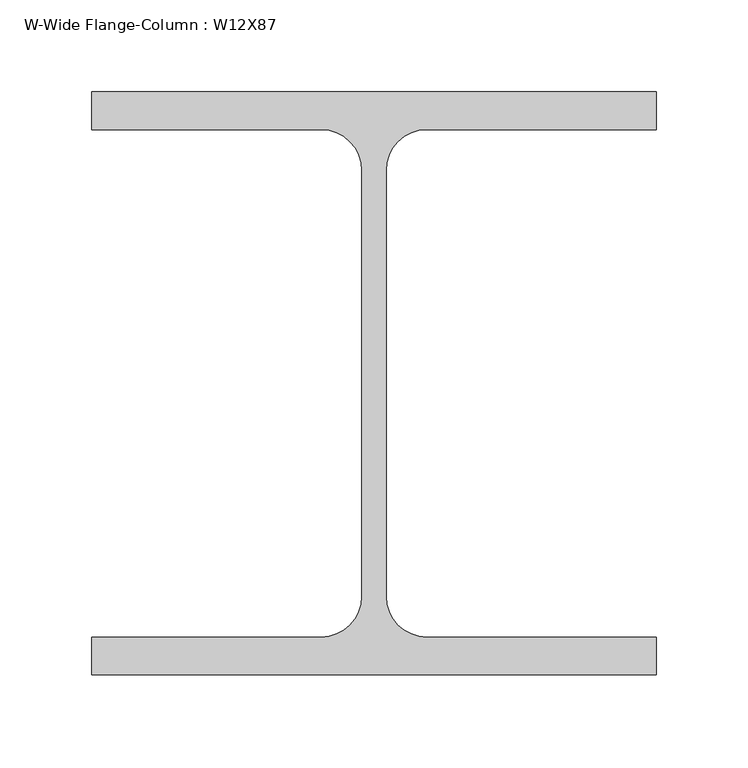
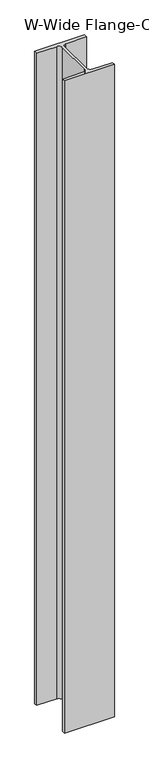
"""IFC4 building model written with IfcOpenShell, lengths in millimetres: column geometry, W-Wide Flange-Column : W12X87."""

from ifc_helpers import new_model, si_unit, point, frame, frame_2d, origin, place, context, project, spatial, polyline, circle_curve, trimmed, segment, composite_curve, outline, extrude, source, transform, mapped, element, save


def w_wide_flange_column_w12x87_8c61926e(model_context):
    return source(origin(), model_context, "Body", "SweptSolid", [
        extrude(outline(composite_curve([segment(polyline([(153.67, 158.75), (153.67, 138.176), (28.829, 138.176)]), True, "CONTINUOUS"), segment(trimmed(circle_curve(frame_2d((28.829, 115.8875)), 22.2885), [point((28.829, 138.176))], [point((6.5405, 115.8875))], True, "CARTESIAN"), True, "CONTINUOUS"), segment(polyline([(6.5405, 115.8875), (6.5405, -115.8875)]), True, "CONTINUOUS"), segment(trimmed(circle_curve(frame_2d((28.829, -115.8875)), 22.2885), [point((6.5405, -115.8875))], [point((28.829, -138.176))], True, "CARTESIAN"), True, "CONTINUOUS"), segment(polyline([(28.829, -138.176), (153.67, -138.176), (153.67, -158.75), (-153.67, -158.75), (-153.67, -138.176), (-28.829, -138.176)]), True, "CONTINUOUS"), segment(trimmed(circle_curve(frame_2d((-28.829, -115.8875)), 22.2885), [point((-28.829, -138.176))], [point((-6.5405, -115.8875))], True, "CARTESIAN"), True, "CONTINUOUS"), segment(polyline([(-6.5405, -115.8875), (-6.5405, 115.8875)]), True, "CONTINUOUS"), segment(trimmed(circle_curve(frame_2d((-28.829, 115.8875)), 22.2885), [point((-6.5405, 115.8875))], [point((-28.829, 138.176))], True, "CARTESIAN"), True, "CONTINUOUS"), segment(polyline([(-28.829, 138.176), (-153.67, 138.176), (-153.67, 158.75), (153.67, 158.75)]), True, "CONTINUOUS")], self_intersect=False)), frame((0.0, 0.0, 13379.45), z_axis=(0.0, 0.0, 1.0), x_axis=(1.0, 0.0, 0.0)), (0.0, 0.0, 1.0), 4248.15),
    ])


if __name__ == "__main__":
    model = new_model("IFC4")
    model_context = context("Model", 3, world=origin())
    ifc_project = project(units=[si_unit("LENGTHUNIT", "METRE", prefix="MILLI")], contexts=[model_context])
    site = spatial("IfcSite", under=ifc_project)
    building = spatial("IfcBuilding", under=site)
    placement = place(None, origin())
    w_wide_flange_column_w12x87_shape = w_wide_flange_column_w12x87_8c61926e(model_context)
    element("IfcColumn", 1, ObjectType="W-Wide Flange-Column : W12X87", at=placement, inside=building, context=model_context, shape_type="MappedRepresentation", body=[
        mapped(w_wide_flange_column_w12x87_shape, transform((0.0, 0.0, 0.0), x_axis=(1.0, 0.0, 0.0), y_axis=(0.0, 1.0, 0.0), z_axis=(0.0, 0.0, 1.0))),
    ])
    save(model, "model.ifc")

# Revit data of these elements
# Type "W-Wide Flange-Column : W12X87"
#   Assembly Code = "B10"
#   W = 87
#   bf = 1' - 0.1"
#   d = 1' - 0 1/2"
#   k = 0' - 1 11/16"
#   kr = 0' - 0.8775"
#   tf = 0' - 0.81"
#   tw = 0' - 0.515"
#   A = 0.177778 SF
#   Structural Material [instance default] = Steel ASTM A992
# Element 1 (IfcColumn, "W-Wide Flange-Column : W12X87")
#   Materials on its faces: "Steel ASTM A992"
# Materials
#   "Steel ASTM A992": class "Metal", colour RGB 199 199 199, transparency 0, Description = "Structural steel 50ksi", Cost = 0
